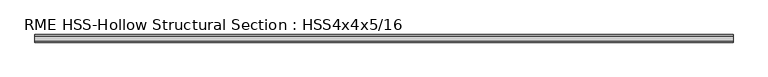
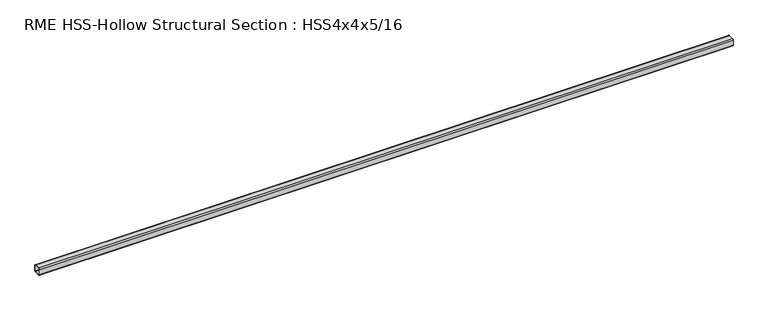
"""IFC4 building model written with IfcOpenShell, lengths in millimetres: member geometry, RME HSS-Hollow Structural Section : HSS4x4x5/16."""

from ifc_helpers import new_model, si_unit, point, frame, frame_2d, origin, place, context, project, spatial, polyline, circle_curve, trimmed, segment, composite_curve, outline, extrude, source, transform, mapped, element, save


def rme_hss_hollow_structural_section_hss4x4x5_16_d95055f5(model_context):
    return source(origin(), model_context, "Body", "SweptSolid", [
        extrude(outline(composite_curve([segment(polyline([(50.8, 36.0172), (50.8, -36.0172)]), True, "CONTINUOUS"), segment(trimmed(circle_curve(frame_2d((36.0172, -36.0172)), 14.7828), [point((50.8, -36.0172))], [point((36.0172, -50.8))], False, "CARTESIAN"), True, "CONTINUOUS"), segment(polyline([(36.0172, -50.8), (-36.0172, -50.8)]), True, "CONTINUOUS"), segment(trimmed(circle_curve(frame_2d((-36.0172, -36.0172)), 14.7828), [point((-36.0172, -50.8))], [point((-50.8, -36.0172))], False, "CARTESIAN"), True, "CONTINUOUS"), segment(polyline([(-50.8, -36.0172), (-50.8, 36.0172)]), True, "CONTINUOUS"), segment(trimmed(circle_curve(frame_2d((-36.0172, 36.0172)), 14.7828), [point((-50.8, 36.0172))], [point((-36.0172, 50.8))], False, "CARTESIAN"), True, "CONTINUOUS"), segment(polyline([(-36.0172, 50.8), (36.0172, 50.8)]), True, "CONTINUOUS"), segment(trimmed(circle_curve(frame_2d((36.0172, 36.0172)), 14.7828), [point((36.0172, 50.8))], [point((50.8, 36.0172))], False, "CARTESIAN"), True, "CONTINUOUS")], self_intersect=False), holes=[composite_curve([segment(trimmed(circle_curve(frame_2d((-36.0172, 36.0172)), 7.3914), [point((-36.0172, 43.4086))], [point((-43.4086, 36.0172))], True, "CARTESIAN"), True, "CONTINUOUS"), segment(polyline([(-43.4086, 36.0172), (-43.4086, -36.0172)]), True, "CONTINUOUS"), segment(trimmed(circle_curve(frame_2d((-36.0172, -36.0172)), 7.3914), [point((-43.4086, -36.0172))], [point((-36.0172, -43.4086))], True, "CARTESIAN"), True, "CONTINUOUS"), segment(polyline([(-36.0172, -43.4086), (36.0172, -43.4086)]), True, "CONTINUOUS"), segment(trimmed(circle_curve(frame_2d((36.0172, -36.0172)), 7.3914), [point((36.0172, -43.4086))], [point((43.4086, -36.0172))], True, "CARTESIAN"), True, "CONTINUOUS"), segment(polyline([(43.4086, -36.0172), (43.4086, 36.0172)]), True, "CONTINUOUS"), segment(trimmed(circle_curve(frame_2d((36.0172, 36.0172)), 7.3914), [point((43.4086, 36.0172))], [point((36.0172, 43.4086))], True, "CARTESIAN"), True, "CONTINUOUS"), segment(polyline([(36.0172, 43.4086), (-36.0172, 43.4086)]), True, "CONTINUOUS")], self_intersect=False)]), frame((-4740.9985659, 0.0, 0.0), z_axis=(1.0, 0.0, 0.0), x_axis=(0.0, 1.0, 0.0)), (0.0, 0.0, 1.0), 9306.1967433),
    ])


if __name__ == "__main__":
    model = new_model("IFC4")
    model_context = context("Model", 3, world=origin())
    ifc_project = project(units=[si_unit("LENGTHUNIT", "METRE", prefix="MILLI")], contexts=[model_context])
    site = spatial("IfcSite", under=ifc_project)
    building = spatial("IfcBuilding", under=site)
    placement = place(None, origin())
    rme_hss_hollow_structural_section_hss4x4x5_16_shape = rme_hss_hollow_structural_section_hss4x4x5_16_d95055f5(model_context)
    element("IfcMember", 1, ObjectType="RME HSS-Hollow Structural Section : HSS4x4x5/16", at=placement, inside=building, context=model_context, shape_type="MappedRepresentation", body=[
        mapped(rme_hss_hollow_structural_section_hss4x4x5_16_shape, transform((0.0, 0.0, 0.0), x_axis=(1.0, 0.0, 0.0), y_axis=(0.0, 1.0, 0.0), z_axis=(0.0, 0.0, 1.0))),
    ])
    save(model, "model.ifc")

# Revit data of these elements
# Type "RME HSS-Hollow Structural Section : HSS4x4x5/16"
#   Nominal Size = "HSS6x4"
#   Assembly Code = "B10"
#   Shape = "Square"
#   W = 14.8
#   Start Extension Calculation [instance default] = 10' - 0"
#   Start Extension [instance default] = -0' - 0 1/2"
#   End Extension Calculation [instance default] = 10' - 0"
#   End Extension [instance default] = -0' - 0 1/2"
#   Ht = 0' - 4"
#   Length [instance default] = 5' - 0"
#   b = 0' - 4"
#   kr = 0' - 0.582"
#   t = 0' - 0.291"
#   A = 0.0284722 SF
#   Structural Material [instance default] = Metal - Steel - ASTM A500 - Grade B - Rectangular and Square
# Element 1 (IfcMember, "RME HSS-Hollow Structural Section : HSS4x4x5/16")
#   Length = 32' - 3.89753"
#   Structural Material = Metal - Steel - ASTM A992
#   Materials on its faces: "Metal - Steel - ASTM A992"
# Materials
#   "Metal - Steel - ASTM A500 - Grade B - Rectangular and Square": class "Metal", colour RGB 255 128 0, transparency 0
#   "Metal - Steel - ASTM A992": class "Metal", colour RGB 255 128 0, transparency 0
